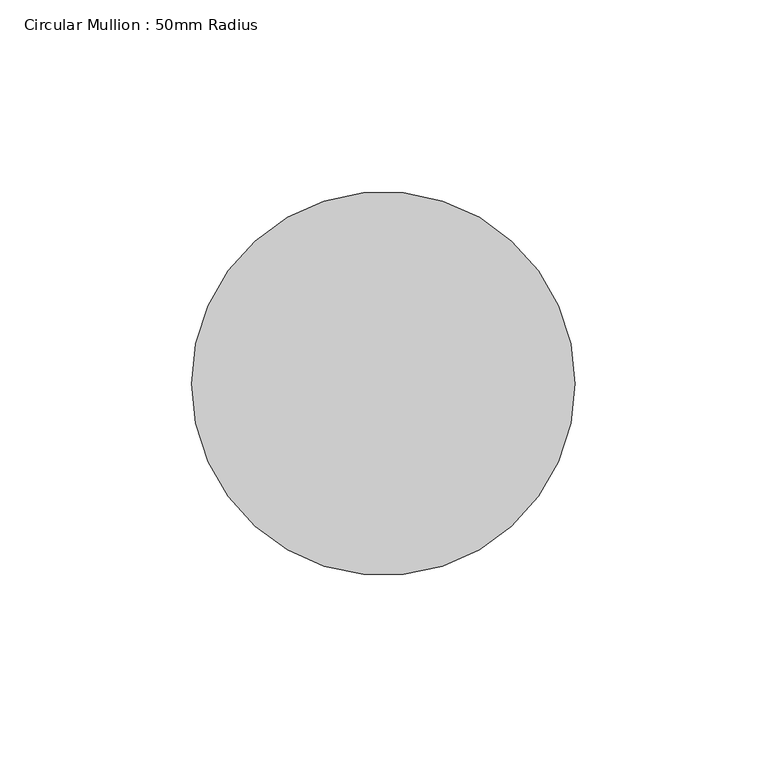
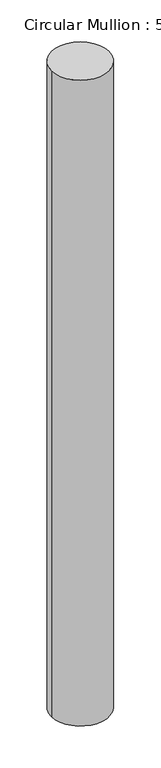
"""IFC4 building model written with IfcOpenShell, lengths in millimetres: member geometry, Circular Mullion : 50mm Radius."""

from ifc_helpers import new_model, si_unit, point, frame, origin, origin_2d, place, context, project, spatial, circle_curve, trimmed, segment, composite_curve, outline, extrude, source, transform, mapped, element, save


def circular_mullion_50mm_radius_310a7bfe(model_context):
    return source(origin(), model_context, "Body", "SweptSolid", [
        extrude(outline(composite_curve([segment(trimmed(circle_curve(origin_2d(), 50.0), [point((50.0, 0.0))], [point((-50.0, 0.0))], False, "CARTESIAN"), True, "CONTINUOUS"), segment(trimmed(circle_curve(origin_2d(), 50.0), [point((-50.0, 0.0))], [point((50.0, 0.0))], False, "CARTESIAN"), True, "CONTINUOUS")], self_intersect=False)), frame((0.0, 0.0, -1180.3120593), z_axis=(0.0, 0.0, 1.0), x_axis=(1.0, 0.0, 0.0)), (0.0, 0.0, 1.0), 1180.3120593),
    ])


if __name__ == "__main__":
    model = new_model("IFC4")
    model_context = context("Model", 3, world=origin())
    ifc_project = project(units=[si_unit("LENGTHUNIT", "METRE", prefix="MILLI")], contexts=[model_context])
    site = spatial("IfcSite", under=ifc_project)
    building = spatial("IfcBuilding", under=site)
    placement = place(None, origin())
    circular_mullion_50mm_radius_shape = circular_mullion_50mm_radius_310a7bfe(model_context)
    element("IfcMember", 1, ObjectType="Circular Mullion : 50mm Radius", at=placement, inside=building, context=model_context, shape_type="MappedRepresentation", body=[
        mapped(circular_mullion_50mm_radius_shape, transform((0.0, 0.0, 0.0), x_axis=(1.0, 0.0, 0.0), y_axis=(0.0, 1.0, 0.0), z_axis=(0.0, 0.0, 1.0))),
    ])
    save(model, "model.ifc")

# Revit data of these elements
# Type "Circular Mullion : 50mm Radius"
#   built-in parameter 1007350 = 0.164042 (stored number, unit not read)
# Element 1 (IfcMember, "Circular Mullion : 50mm Radius")
#   Materials on its faces: "Aluminium"
# Materials
#   "Aluminium": class "Metal", colour RGB 247 247 247, transparency 0, Description = "Aluminium 6061", Cost = 0
